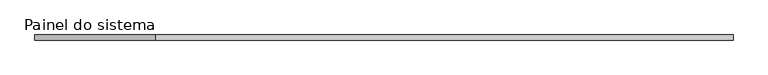
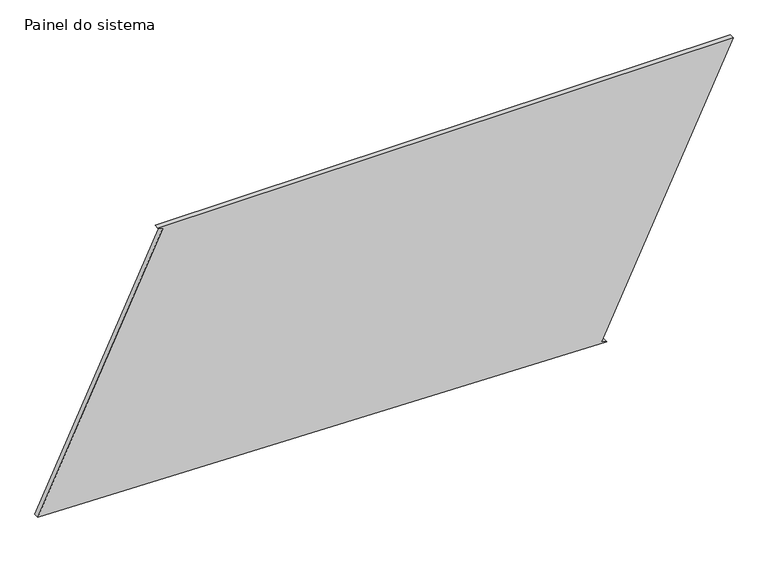
"""IFC4 building model written with IfcOpenShell, lengths in millimetres: plate geometry, Painel do sistema : Envidraçado."""

from ifc_helpers import new_model, si_unit, frame, origin, place, context, project, spatial, polyline, outline, extrude, source, transform, mapped, element, save


def painel_do_sistema_7bcbdab4(model_context):
    return source(origin(), model_context, "Body", "SweptSolid", [
        extrude(outline(polyline([(0.0, 1085.0499125), (10.7698497, 1062.488655), (1359.3571306, 1706.2507456), (1359.3571306, -1116.7622695), (1348.587281, -1094.201012), (66.4327426, -1706.2507456), (0.0, 1085.0499125)])), frame((0.0, 24.5, 0.0), z_axis=(0.0, 1.0, 0.0), x_axis=(0.0, 0.0, 1.0)), (0.0, 0.0, 1.0), 25.0),
    ])


if __name__ == "__main__":
    model = new_model("IFC4")
    model_context = context("Model", 3, world=origin())
    ifc_project = project(units=[si_unit("LENGTHUNIT", "METRE", prefix="MILLI")], contexts=[model_context])
    site = spatial("IfcSite", under=ifc_project)
    building = spatial("IfcBuilding", under=site)
    placement = place(None, origin())
    painel_do_sistema_shape = painel_do_sistema_7bcbdab4(model_context)
    element("IfcPlate", 1, ObjectType="Painel do sistema : Envidraçado", at=placement, inside=building, context=model_context, shape_type="MappedRepresentation", body=[
        mapped(painel_do_sistema_shape, transform((0.0, 0.0, 0.0), x_axis=(1.0, 0.0, 0.0), y_axis=(0.0, 1.0, 0.0), z_axis=(0.0, 0.0, 1.0))),
    ])
    save(model, "model.ifc")

# Revit data of these elements
# Type "Painel do sistema : Envidraçado"
#   Construction Type Id = "GSP4R"
#   Analytic Construction = "Vidraça única Pilkington 1/8 pol"
#   Visual Light Transmittance = 0.9
#   Solar Heat Gain Coefficient = 0.86
#   Heat Transfer Coefficient (U) = 6.7069 W/(m²·K)
# Element 1 (IfcPlate, "Painel do sistema : Envidraçado")
#   Materials on its faces: "Vidro"
# Materials
#   "Vidro": class "Vidro", colour RGB 0 128 192, transparency 0.9, Description = "Vidro de sílica", Cost = 0
